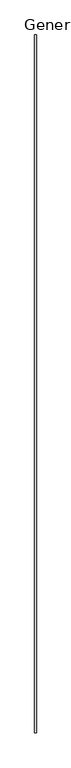
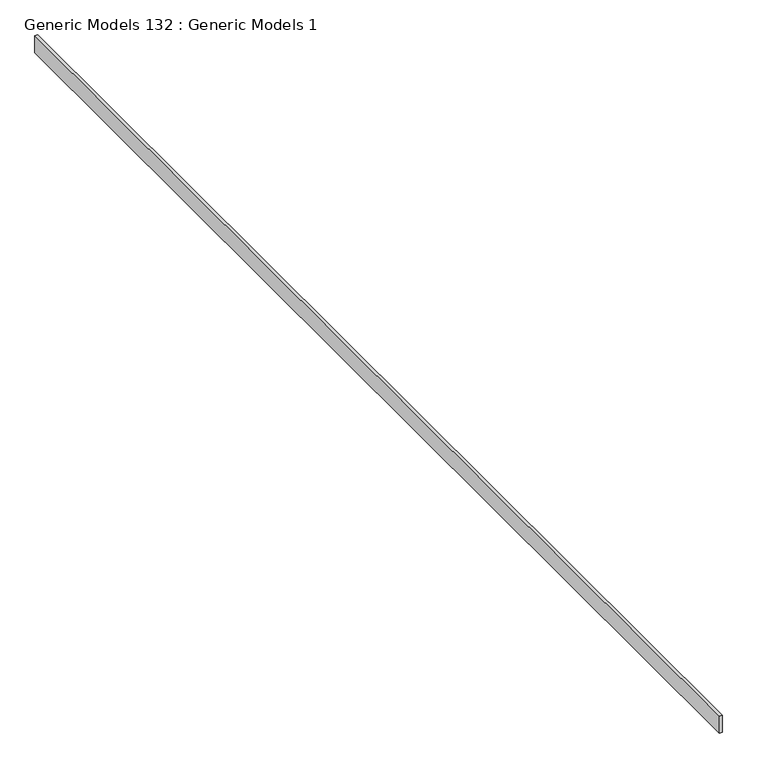
"""IFC4 building model written with IfcOpenShell, lengths in millimetres: proxy geometry, Generic Models 132 : Generic Models 1."""

from ifc_helpers import new_model, si_unit, frame, origin, place, context, project, spatial, polyline, outline, extrude, source, transform, mapped, element, save


def generic_models_132_generic_models_1_bb5e9510(model_context):
    return source(origin(), model_context, "Body", "SweptSolid", [
        extrude(outline(polyline([(7095.9513704, 11981.8769662), (7140.4013704, 11981.8769662), (7140.4013704, -7068.1230338), (7095.9513704, -7068.1230338), (7095.9513704, 11981.8769662)])), frame((0.0, 0.0, 126485.396), z_axis=(0.0, 0.0, 1.0), x_axis=(1.0, 0.0, 0.0)), (0.0, 0.0, 1.0), 285.75),
    ])


if __name__ == "__main__":
    model = new_model("IFC4")
    model_context = context("Model", 3, world=origin())
    ifc_project = project(units=[si_unit("LENGTHUNIT", "METRE", prefix="MILLI")], contexts=[model_context])
    site = spatial("IfcSite", under=ifc_project)
    building = spatial("IfcBuilding", under=site)
    placement = place(None, origin())
    generic_models_132_generic_models_1_shape = generic_models_132_generic_models_1_bb5e9510(model_context)
    element("IfcBuildingElementProxy", 1, Name="Generic Models 132 : Generic Models 1", ObjectType="Generic Models 132 : Generic Models 1", at=placement, inside=building, context=model_context, shape_type="MappedRepresentation", body=[
        mapped(generic_models_132_generic_models_1_shape, transform((0.0, 0.0, 0.0), x_axis=(1.0, 0.0, 0.0), y_axis=(0.0, 1.0, 0.0), z_axis=(0.0, 0.0, 1.0))),
    ])
    save(model, "model.ifc")

# Revit data of these elements
# Element 1 (IfcBuildingElementProxy, "Generic Models 132 : Generic Models 1")
#   Materials on its faces: "_STRUCTURAL MEMBER (SEE STRUCT. DWGS)"
# Materials
#   "_STRUCTURAL MEMBER (SEE STRUCT. DWGS)": class "Generic", colour RGB 209 182 141, transparency 0, Cost = 0
